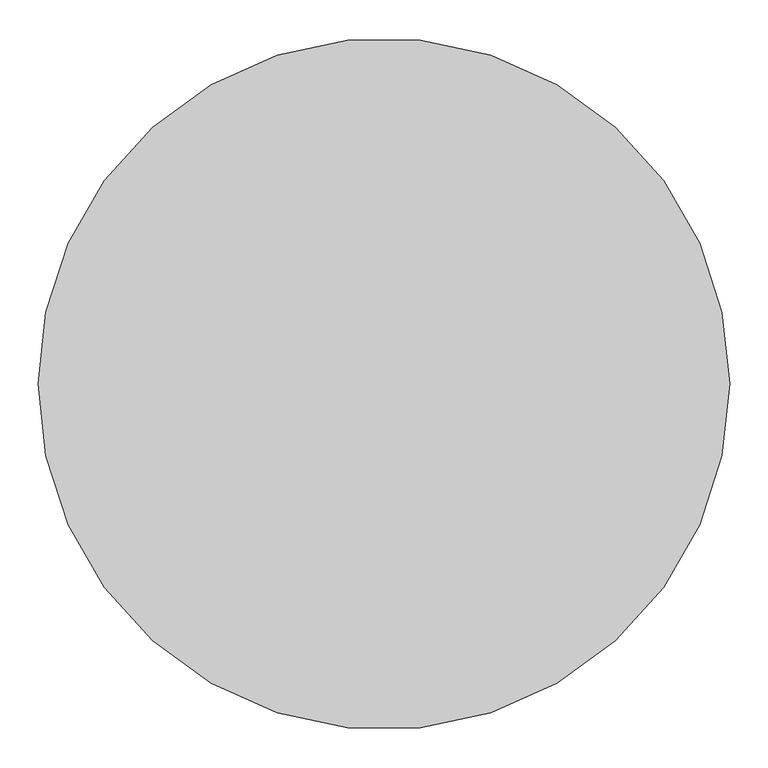
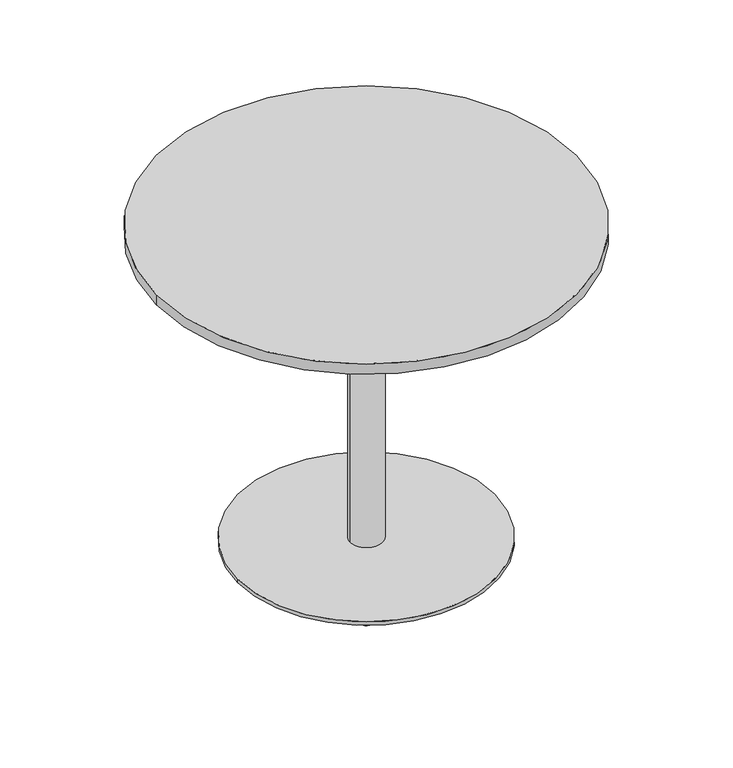
"""IFC4 building model written with IfcOpenShell, lengths in millimetres: furniture geometry, Furniture_Office-Desks&Tables_Kinnarps_MULTICOM-Round-meeting-table-900mm_U-MCZZM9RN : Furniture_Office-Desks&Tables_Kinnarps_MULTICOM-Round-meeting-table-900mm_U-MCZZM9RN."""

from ifc_helpers import new_model, si_unit, point, frame, frame_2d, origin, origin_with_axes, origin_2d, place, context, project, spatial, circle_curve, trimmed, segment, composite_curve, outline, extrude, source, transform, mapped, element, save


def furniture_2aac9d90(model_context):
    return source(origin(), model_context, "Body", "SweptSolid", [
        extrude(outline(composite_curve([segment(trimmed(circle_curve(frame_2d((-255.0001328, 0.0)), 12.5), [point((-267.5001328, 0.0))], [point((-242.5001328, 0.0))], False, "CARTESIAN"), True, "CONTINUOUS"), segment(trimmed(circle_curve(frame_2d((-255.0001328, 0.0)), 12.5), [point((-242.5001328, 0.0))], [point((-267.5001328, 0.0))], False, "CARTESIAN"), True, "CONTINUOUS")], self_intersect=False)), origin_with_axes(), (0.0, 0.0, 1.0), 6.0),
        extrude(outline(composite_curve([segment(trimmed(circle_curve(frame_2d((-127.5000664, 220.7093513)), 12.5), [point((-140.0000664, 220.7093513))], [point((-115.0000664, 220.7093513))], False, "CARTESIAN"), True, "CONTINUOUS"), segment(trimmed(circle_curve(frame_2d((-127.5000664, 220.7093513)), 12.5), [point((-115.0000664, 220.7093513))], [point((-140.0000664, 220.7093513))], False, "CARTESIAN"), True, "CONTINUOUS")], self_intersect=False)), origin_with_axes(), (0.0, 0.0, 1.0), 6.0),
        extrude(outline(composite_curve([segment(trimmed(circle_curve(frame_2d((127.5000664, 220.7093513)), 12.5), [point((115.0000664, 220.7093513))], [point((140.0000664, 220.7093513))], False, "CARTESIAN"), True, "CONTINUOUS"), segment(trimmed(circle_curve(frame_2d((127.5000664, 220.7093513)), 12.5), [point((140.0000664, 220.7093513))], [point((115.0000664, 220.7093513))], False, "CARTESIAN"), True, "CONTINUOUS")], self_intersect=False)), origin_with_axes(), (0.0, 0.0, 1.0), 6.0),
        extrude(outline(composite_curve([segment(trimmed(circle_curve(frame_2d((255.0001777, 0.0)), 12.5), [point((242.5001777, 0.0))], [point((267.5001777, 0.0))], False, "CARTESIAN"), True, "CONTINUOUS"), segment(trimmed(circle_curve(frame_2d((255.0001777, 0.0)), 12.5), [point((267.5001777, 0.0))], [point((242.5001777, 0.0))], False, "CARTESIAN"), True, "CONTINUOUS")], self_intersect=False)), origin_with_axes(), (0.0, 0.0, 1.0), 6.0),
        extrude(outline(composite_curve([segment(trimmed(circle_curve(frame_2d((-127.5000664, -220.7093513)), 12.5), [point((-140.0000664, -220.7093513))], [point((-115.0000664, -220.7093513))], False, "CARTESIAN"), True, "CONTINUOUS"), segment(trimmed(circle_curve(frame_2d((-127.5000664, -220.7093513)), 12.5), [point((-115.0000664, -220.7093513))], [point((-140.0000664, -220.7093513))], False, "CARTESIAN"), True, "CONTINUOUS")], self_intersect=False)), origin_with_axes(), (0.0, 0.0, 1.0), 6.0),
        extrude(outline(composite_curve([segment(trimmed(circle_curve(frame_2d((127.7500664, -220.7093513)), 12.5), [point((115.2500664, -220.7093513))], [point((140.2500664, -220.7093513))], False, "CARTESIAN"), True, "CONTINUOUS"), segment(trimmed(circle_curve(frame_2d((127.7500664, -220.7093513)), 12.5), [point((140.2500664, -220.7093513))], [point((115.2500664, -220.7093513))], False, "CARTESIAN"), True, "CONTINUOUS")], self_intersect=False)), origin_with_axes(), (0.0, 0.0, 1.0), 6.0),
        extrude(outline(composite_curve([segment(trimmed(circle_curve(origin_2d(), 35.0), [point((35.0, 0.0))], [point((-35.0, 0.0))], False, "CARTESIAN"), True, "CONTINUOUS"), segment(trimmed(circle_curve(origin_2d(), 35.0), [point((-35.0, 0.0))], [point((35.0, 0.0))], False, "CARTESIAN"), True, "CONTINUOUS")], self_intersect=False)), frame((0.0, 0.0, 14.0), z_axis=(0.0, 0.0, 1.0), x_axis=(1.0, 0.0, 0.0)), (0.0, 0.0, 1.0), 683.0),
        extrude(outline(composite_curve([segment(trimmed(circle_curve(origin_2d(), 275.0), [point((275.0, 0.0))], [point((-275.0, 0.0))], False, "CARTESIAN"), True, "CONTINUOUS"), segment(trimmed(circle_curve(origin_2d(), 275.0), [point((-275.0, 0.0))], [point((275.0, 0.0))], False, "CARTESIAN"), True, "CONTINUOUS")], self_intersect=False)), frame((0.0, 0.0, 6.0), z_axis=(0.0, 0.0, 1.0), x_axis=(1.0, 0.0, 0.0)), (0.0, 0.0, 1.0), 8.0),
        extrude(outline(composite_curve([segment(trimmed(circle_curve(origin_2d(), 450.0), [point((450.0, 0.0))], [point((-450.0, 0.0))], False, "CARTESIAN"), True, "CONTINUOUS"), segment(trimmed(circle_curve(origin_2d(), 450.0), [point((-450.0, 0.0))], [point((450.0, 0.0))], False, "CARTESIAN"), True, "CONTINUOUS")], self_intersect=False)), frame((0.0, 0.0, 697.0), z_axis=(0.0, 0.0, 1.0), x_axis=(1.0, 0.0, 0.0)), (0.0, 0.0, 1.0), 23.0),
    ])


if __name__ == "__main__":
    model = new_model("IFC4")
    model_context = context("Model", 3, world=origin())
    ifc_project = project(units=[si_unit("LENGTHUNIT", "METRE", prefix="MILLI")], contexts=[model_context])
    site = spatial("IfcSite", under=ifc_project)
    building = spatial("IfcBuilding", under=site)
    placement = place(None, origin())
    furniture_shape = furniture_2aac9d90(model_context)
    element("IfcFurniture", 1, ObjectType="Furniture_Office-Desks&Tables_Kinnarps_MULTICOM-Round-meeting-table-900mm_U-MCZZM9RN : Furniture_Office-Desks&Tables_Kinnarps_MULTICOM-Round-meeting-table-900mm_U-MCZZM9RN", at=placement, inside=building, context=model_context, shape_type="MappedRepresentation", body=[
        mapped(furniture_shape, transform((0.0, 0.0, 0.0), x_axis=(1.0, 0.0, 0.0), y_axis=(0.0, 1.0, 0.0), z_axis=(0.0, 0.0, 1.0))),
    ])
    save(model, "model.ifc")

# Revit data of these elements
# Type "Furniture_Office-Desks&Tables_Kinnarps_MULTICOM-Round-meeting-table-900mm_U-MCZZM9RN : Furniture_Office-Desks&Tables_Kinnarps_MULTICOM-Round-meeting-table-900mm_U-MCZZM9RN"
#   Youtube clip = "https://www.youtube.com/watch?v=ibDSYpyJ4ZM"
#   Weight Net (Kg) = ""
#   WarrantyStartDate = ""
#   WarrantyDuration = ""
#   Uniformat II Description = ""
#   Uniformat II Code = ""
#   Uniclass 2015 Name = ""
#   Uniclass 2015 Code = ""
#   Uniclass 2.0 Description = "Desks, Tables And Worktops"
#   Uniclass 2.0 Code = "PR-31-22"
#   Uniclass 1.4 Description = "Conference room furniture"
#   Uniclass 1.4 Code = "L8536"
#   URL = "https://bimobject.com/kinnarps/product/u-mczzm9rn"
#   UNSPSC Code = ""
#   UNSPSC Category = "Furniture and Furnishings"
#   TypeName = "U-MCZZM9RN"
#   Technical description = "http://www.kinnarps.com/en/International/ProductsInspiration/Office/ConferenceTables/Product/?prodid=305786#"
#   TagNumber = ""
#   Size = ""
#   SerialNumber = ""
#   Region South America = "None"
#   Region Oceania = "None"
#   Region North America = "None"
#   Region Middle East = "None"
#   Region Europe = "AD, AL, AT, AX, BA, BE, BG, BY, CH, CY, CZ, DE, DK, EE, ES, FI, FO, FR, GB, GG, GI, GR, HR, HU, IE, IM, IS, IT, JE, LI, LT, LU, LV, MC, MD, ME, MK, MT, NL, NO, PL, PT, RO, RS, RU, SE, SI, SJ, SK, SM, UA, VA"
#   Region Asia = "None"
#   Region Antarctica = "None"
#   Region Africa = "None"
#   QR code = "http://bimobject.com/kinnarps/product/U-MCZZM9RN"
#   Product url = "http://www.kinnarps.com/en/International/ProductsInspiration/Office/ConferenceTables/Product/?prodid=305786"
#   Product identifier = "kinnarps.bimobject.com/U-MCZZM9RN"
#   Product group = "MULTICOM"
#   Product family = "Conference tables"
#   Product data url = "https://bimobject.com/kinnarps/product/U-MCZZM9RN"
#   Product certification = ""
#   Product SKU = "U-MCZZM9RN"
#   Product Guid = "8fde862c-6a63-4273-8c9c-abfa813065ee"
#   Omniclass = "23.40.70.14.64.11"
#   OmniClass Description = ""
#   OmniClass Code = ""
#   Name of the object = "MULTICOM U-MCZZM9RN"
#   NBS Reference Description = "Desks, Tables And Worktops"
#   NBS Reference Code = "31-22"
#   NBS Reference = "31-22"
#   Model = "MULTICOM U-MCZZM9RN"
#   Material secondary = ""
#   Material main = ""
#   Material = ""
#   Masterformat 2014 Description = "Furnishings"
#   Masterformat 2014 Code = "12 00 00"
#   Manufacturer name = "Kinnarps"
#   Manufacturer country = "Sweden"
#   Manufacturer URL = "http://www.kinnarps.com"
#   Manufacturer = "Kinnarps"
#   InstallationDate = ""
#   Installation instructions = "http://www.kinnarps.com/en/International/ProductsInspiration/Office/ConferenceTables/Product/?prodid=305786#"
#   IFC Classification = "Furniture"
#   Grade = ""
#   Finish = ""
#   Features = ""
#   Extidentifier = ""
#   EAN code = ""
#   Design country = "Sweden"
#   Date of publishing = "1/15/2014"
#   Created on = ""
#   Created by = ""
#   ConnectionType = ""
#   Colour = ""
#   COBIe Type Category = ""
#   Brand url = "http://www.kinnarps.com/"
#   Barcode = ""
#   BIMobject QR code url = "http://kinnarps.bimobject.com/U-MCZZM9RN"
#   BIMobject Category = "Office Desks & Tables"
#   AssetIdentifier = ""
#   AccessibilityPerformance = ""
#   Width (mm) = 900 mm
#   Table Top Radius = 450 mm
#   Offset = 0 mm
#   Nominal width = 900 mm
#   Nominal height = 720 mm
#   Height (mm) = 720 mm
#   Depth (mm) = 900 mm
#   Edition number = 2
#   Table Top [instance default] = Kinnarps-Laminate-Beech
#   Table Leg [instance default] = Kinnarps-Metal-White
#   Default Elevation = 0
# Element 1 (IfcFurniture, "Furniture_Office-Desks&Tables_Kinnarps_MULTICOM-Round-meeting-table-900mm_U-MCZZM9RN : Furniture_Office-Desks&Tables_Kinnarps_MULTICOM-Round-meeting-table-900mm_U-MCZZM9RN")
#   Table Top = Kinnarps-Laminate-White
#   Materials on its faces: "Kinnarps-Plastic-Black", "Kinnarps-Metal-White", "Kinnarps-Laminate-White"
# Materials
#   "Kinnarps-Laminate-Beech": class "Miscellaneous", colour RGB 174 140 106, transparency 0
#   "Kinnarps-Metal-White": class "Miscellaneous", colour RGB 255 255 255, transparency 0
#   "Kinnarps-Plastic-Black": class "Miscellaneous", colour RGB 0 0 0, transparency 0
#   "Kinnarps-Laminate-White": class "Miscellaneous", colour RGB 255 255 255, transparency 0
